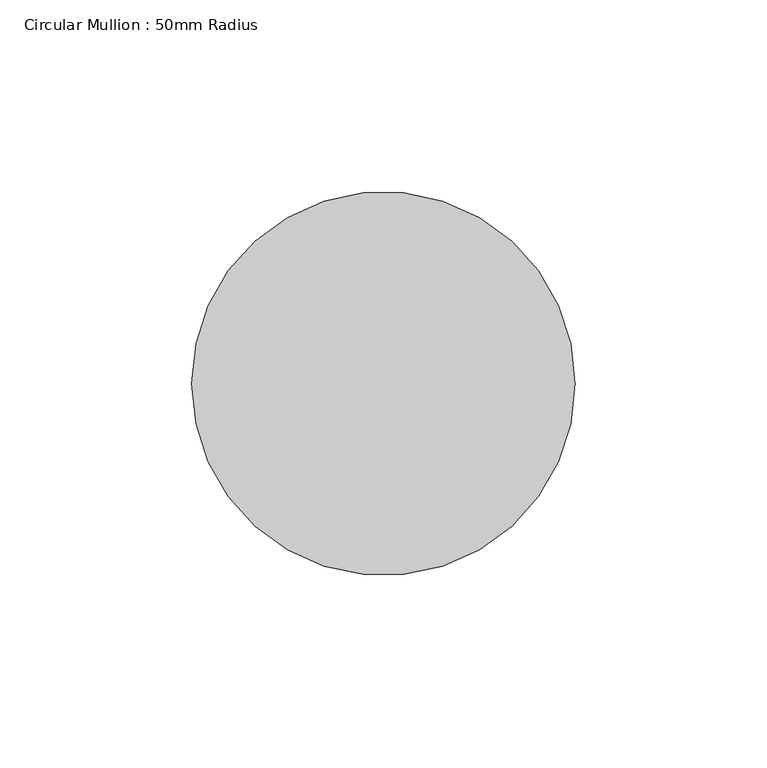
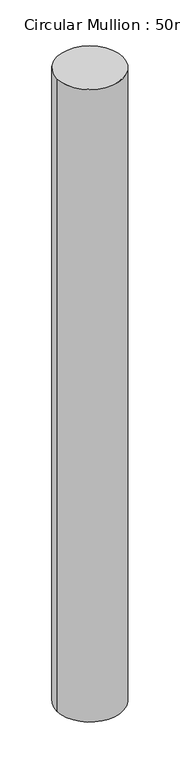
"""IFC4 building model written with IfcOpenShell, lengths in millimetres: member geometry, Circular Mullion : 50mm Radius."""

from ifc_helpers import new_model, si_unit, point, frame, origin, origin_2d, place, context, project, spatial, circle_curve, trimmed, segment, composite_curve, outline, extrude, source, transform, mapped, element, save


def circular_mullion_50mm_radius_f572cb39(model_context):
    return source(origin(), model_context, "Body", "SweptSolid", [
        extrude(outline(composite_curve([segment(trimmed(circle_curve(origin_2d(), 50.0), [point((50.0, 0.0))], [point((-50.0, 0.0))], False, "CARTESIAN"), True, "CONTINUOUS"), segment(trimmed(circle_curve(origin_2d(), 50.0), [point((-50.0, 0.0))], [point((50.0, 0.0))], False, "CARTESIAN"), True, "CONTINUOUS")], self_intersect=False)), frame((0.0, 0.0, -1016.7631045), z_axis=(0.0, 0.0, 1.0), x_axis=(1.0, 0.0, 0.0)), (0.0, 0.0, 1.0), 1016.7631045),
    ])


if __name__ == "__main__":
    model = new_model("IFC4")
    model_context = context("Model", 3, world=origin())
    ifc_project = project(units=[si_unit("LENGTHUNIT", "METRE", prefix="MILLI")], contexts=[model_context])
    site = spatial("IfcSite", under=ifc_project)
    building = spatial("IfcBuilding", under=site)
    placement = place(None, origin())
    circular_mullion_50mm_radius_shape = circular_mullion_50mm_radius_f572cb39(model_context)
    element("IfcMember", 1, ObjectType="Circular Mullion : 50mm Radius", at=placement, inside=building, context=model_context, shape_type="MappedRepresentation", body=[
        mapped(circular_mullion_50mm_radius_shape, transform((0.0, 0.0, 0.0), x_axis=(1.0, 0.0, 0.0), y_axis=(0.0, 1.0, 0.0), z_axis=(0.0, 0.0, 1.0))),
    ])
    save(model, "model.ifc")

# Revit data of these elements
# Type "Circular Mullion : 50mm Radius"
#   built-in parameter 1007350 = 0.164042 (stored number, unit not read)
# Element 1 (IfcMember, "Circular Mullion : 50mm Radius")
#   Materials on its faces: "Aluminium"
# Materials
#   "Aluminium": class "Metal", colour RGB 247 247 247, transparency 0, Description = "Aluminium 6061", Cost = 0
